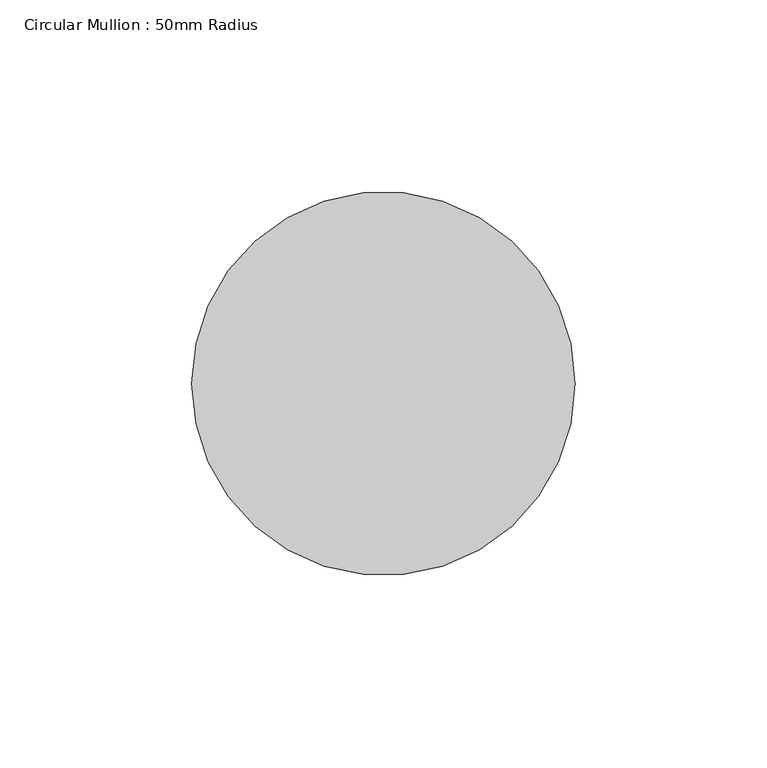
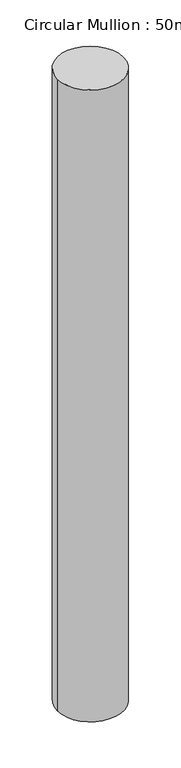
"""IFC4 building model written with IfcOpenShell, lengths in millimetres: member geometry, Circular Mullion : 50mm Radius."""

from ifc_helpers import new_model, si_unit, point, frame, origin, origin_2d, place, context, project, spatial, circle_curve, trimmed, segment, composite_curve, outline, extrude, source, transform, mapped, element, save


def circular_mullion_50mm_radius_af8b6d01(model_context):
    return source(origin(), model_context, "Body", "SweptSolid", [
        extrude(outline(composite_curve([segment(trimmed(circle_curve(origin_2d(), 50.0), [point((50.0, 0.0))], [point((-50.0, 0.0))], False, "CARTESIAN"), True, "CONTINUOUS"), segment(trimmed(circle_curve(origin_2d(), 50.0), [point((-50.0, 0.0))], [point((50.0, 0.0))], False, "CARTESIAN"), True, "CONTINUOUS")], self_intersect=False)), frame((0.0, 0.0, -1009.6313709), z_axis=(0.0, 0.0, 1.0), x_axis=(1.0, 0.0, 0.0)), (0.0, 0.0, 1.0), 1009.6313709),
    ])


if __name__ == "__main__":
    model = new_model("IFC4")
    model_context = context("Model", 3, world=origin())
    ifc_project = project(units=[si_unit("LENGTHUNIT", "METRE", prefix="MILLI")], contexts=[model_context])
    site = spatial("IfcSite", under=ifc_project)
    building = spatial("IfcBuilding", under=site)
    placement = place(None, origin())
    circular_mullion_50mm_radius_shape = circular_mullion_50mm_radius_af8b6d01(model_context)
    element("IfcMember", 1, ObjectType="Circular Mullion : 50mm Radius", at=placement, inside=building, context=model_context, shape_type="MappedRepresentation", body=[
        mapped(circular_mullion_50mm_radius_shape, transform((0.0, 0.0, 0.0), x_axis=(1.0, 0.0, 0.0), y_axis=(0.0, 1.0, 0.0), z_axis=(0.0, 0.0, 1.0))),
    ])
    save(model, "model.ifc")

# Revit data of these elements
# Type "Circular Mullion : 50mm Radius"
#   built-in parameter 1007350 = 0.164042 (stored number, unit not read)
# Element 1 (IfcMember, "Circular Mullion : 50mm Radius")
#   Materials on its faces: "Aluminium"
# Materials
#   "Aluminium": class "Metal", colour RGB 247 247 247, transparency 0, Description = "Aluminium 6061", Cost = 0
